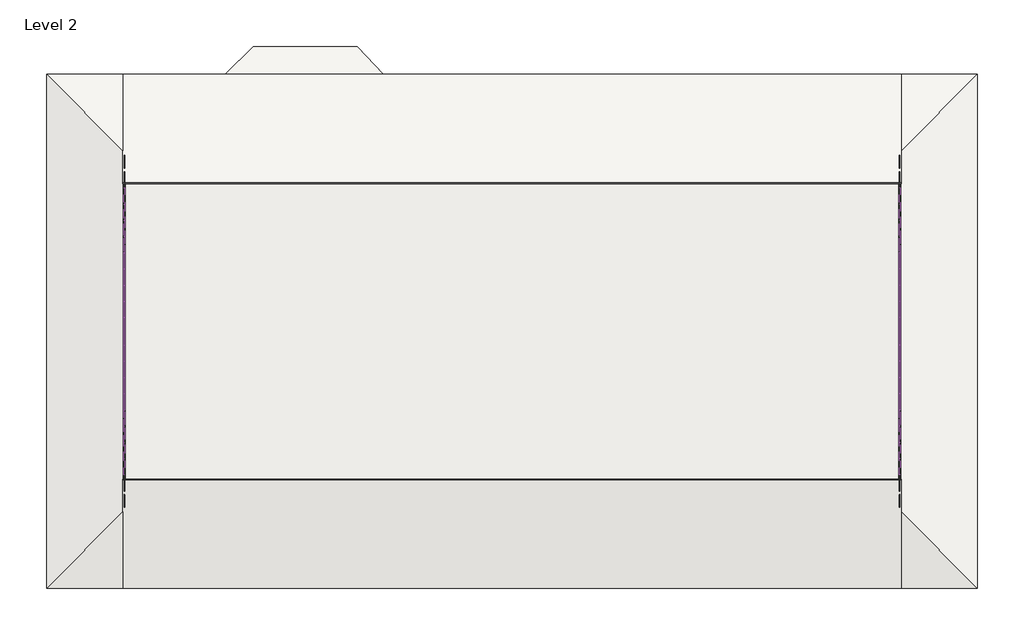
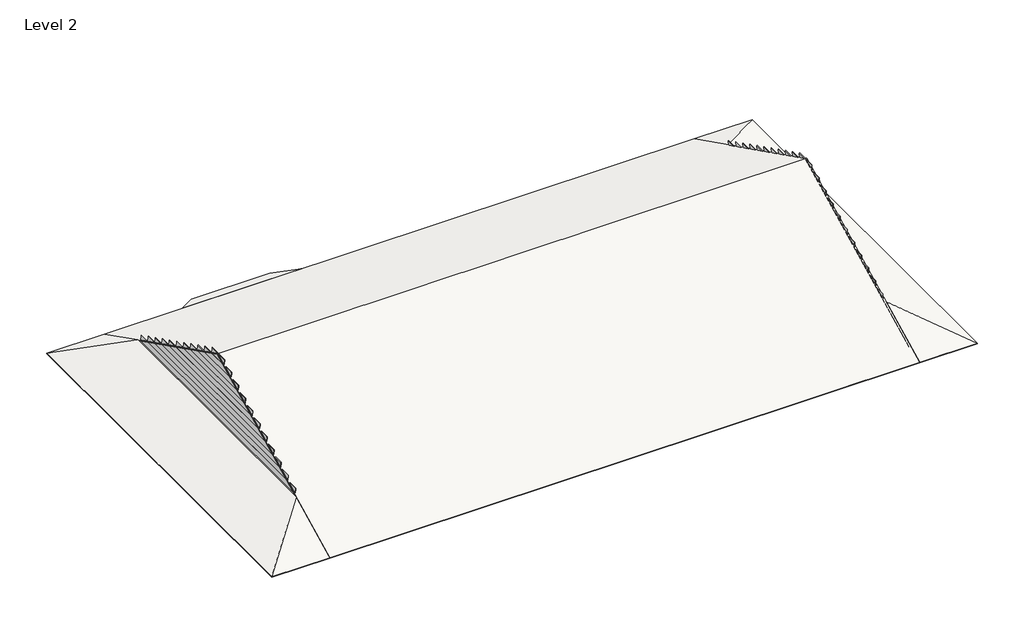
# One storey: 22 proxies, 4 roofs, 2 walls, 1 covering.
"""IFC4 building model written with IfcOpenShell, lengths in millimetres."""

from ifc_helpers import new_model, si_unit, frame, origin, place, context, project, spatial, polyline, outline, extrude, faceted_brep, element, save

model = new_model("IFC4")

# Units and contexts
model_context = context("Model", 3, world=origin())
ifc_project = project(units=[si_unit("LENGTHUNIT", "METRE", prefix="MILLI")], contexts=[model_context])

# Site, building, storey
site = spatial("IfcSite", under=ifc_project)
building = spatial("IfcBuilding", under=site)
storey = spatial("IfcBuildingStorey", under=building, Name="Level 2", Elevation=2768.6)

# Proxies
placement = place(None, origin())
element("IfcBuildingElementProxy", 1, Name="Wall Sweeps", at=placement, inside=storey, context=model_context, shape_type="SweptSolid", body=[
    extrude(outline(polyline([(0.0, -10.0), (0.0, 0.0), (7721.6, 0.0), (7721.6, -10.0), (0.0, -10.0)])), frame((468.8525114, 3886.9284114, 3659.1151454), z_axis=(-0.08859633935570814, 0.0, 0.9960676124906221), x_axis=(0.0, -1.0, 0.0)), (0.0, 0.0, 1.0), 160.0),
])
element("IfcBuildingElementProxy", 2, Name="Wall Sweeps", at=placement, inside=storey, context=model_context, shape_type="SweptSolid", body=[
    extrude(outline(polyline([(0.0, -10.0), (0.0, 0.0), (7010.4, 0.0), (7010.4, -10.0), (0.0, -10.0)])), frame((468.8525114, 3531.3284114, 3836.9151454), z_axis=(-0.08859633935570814, 0.0, 0.9960676124906221), x_axis=(0.0, -1.0, 0.0)), (0.0, 0.0, 1.0), 160.0),
])
element("IfcBuildingElementProxy", 3, Name="Wall Sweeps", at=placement, inside=storey, context=model_context, shape_type="SweptSolid", body=[
    extrude(outline(polyline([(0.0, -10.0), (0.0, 0.0), (6299.2, 0.0), (6299.2, -10.0), (0.0, -10.0)])), frame((468.8525114, 3175.7284114, 4014.7151454), z_axis=(-0.08859633935570814, 0.0, 0.9960676124906221), x_axis=(0.0, -1.0, 0.0)), (0.0, 0.0, 1.0), 160.0),
])
element("IfcBuildingElementProxy", 4, Name="Wall Sweeps", at=placement, inside=storey, context=model_context, shape_type="SweptSolid", body=[
    extrude(outline(polyline([(0.0, -10.0), (0.0, 0.0), (5588.0, 0.0), (5588.0, -10.0), (0.0, -10.0)])), frame((468.8525114, 2820.1284114, 4192.5151454), z_axis=(-0.08859633935570814, 0.0, 0.9960676124906221), x_axis=(0.0, -1.0, 0.0)), (0.0, 0.0, 1.0), 160.0),
])
element("IfcBuildingElementProxy", 5, Name="Wall Sweeps", at=placement, inside=storey, context=model_context, shape_type="SweptSolid", body=[
    extrude(outline(polyline([(0.0, -10.0), (0.0, 0.0), (4876.8, 0.0), (4876.8, -10.0), (0.0, -10.0)])), frame((468.8525114, 2464.5284114, 4370.3151454), z_axis=(-0.08859633935570814, 0.0, 0.9960676124906221), x_axis=(0.0, -1.0, 0.0)), (0.0, 0.0, 1.0), 160.0),
])
element("IfcBuildingElementProxy", 6, Name="Wall Sweeps", at=placement, inside=storey, context=model_context, shape_type="SweptSolid", body=[
    extrude(outline(polyline([(0.0, -10.0), (0.0, 0.0), (4165.6, 0.0), (4165.6, -10.0), (0.0, -10.0)])), frame((468.8525114, 2108.9284114, 4548.1151454), z_axis=(-0.08859633935570814, 0.0, 0.9960676124906221), x_axis=(0.0, -1.0, 0.0)), (0.0, 0.0, 1.0), 160.0),
])
element("IfcBuildingElementProxy", 7, Name="Wall Sweeps", at=placement, inside=storey, context=model_context, shape_type="SweptSolid", body=[
    extrude(outline(polyline([(0.0, -10.0), (0.0, 0.0), (3454.4, 0.0), (3454.4, -10.0), (0.0, -10.0)])), frame((468.8525114, 1753.3284114, 4725.9151454), z_axis=(-0.08859633935570814, 0.0, 0.9960676124906221), x_axis=(0.0, -1.0, 0.0)), (0.0, 0.0, 1.0), 160.0),
])
element("IfcBuildingElementProxy", 8, Name="Wall Sweeps", at=placement, inside=storey, context=model_context, shape_type="SweptSolid", body=[
    extrude(outline(polyline([(0.0, -10.0000001), (0.0, 0.0), (7721.6, 0.0), (7721.6, -10.0000001), (0.0, -10.0000001)])), frame((-16554.1214933, 3886.9284114, 3658.229182), z_axis=(0.08859633935570814, 0.0, 0.9960676124906221), x_axis=(0.0, -1.0, 0.0)), (0.0, 0.0, 1.0), 160.0),
])
element("IfcBuildingElementProxy", 9, Name="Wall Sweeps", at=placement, inside=storey, context=model_context, shape_type="SweptSolid", body=[
    extrude(outline(polyline([(0.0, -10.0000001), (0.0, 0.0), (7010.4, 0.0), (7010.4, -10.0000001), (0.0, -10.0000001)])), frame((-16554.1214933, 3531.3284114, 3836.029182), z_axis=(0.08859633935570814, 0.0, 0.9960676124906221), x_axis=(0.0, -1.0, 0.0)), (0.0, 0.0, 1.0), 160.0),
])
element("IfcBuildingElementProxy", 10, Name="Wall Sweeps", at=placement, inside=storey, context=model_context, shape_type="SweptSolid", body=[
    extrude(outline(polyline([(0.0, -10.0000001), (0.0, 0.0), (6299.2, 0.0), (6299.2, -10.0000001), (0.0, -10.0000001)])), frame((-16554.1214933, 3175.7284114, 4013.829182), z_axis=(0.08859633935570814, 0.0, 0.9960676124906221), x_axis=(0.0, -1.0, 0.0)), (0.0, 0.0, 1.0), 160.0),
])
element("IfcBuildingElementProxy", 11, Name="Wall Sweeps", at=placement, inside=storey, context=model_context, shape_type="SweptSolid", body=[
    extrude(outline(polyline([(0.0, -10.0000001), (0.0, 0.0), (5588.0, 0.0), (5588.0, -10.0000001), (0.0, -10.0000001)])), frame((-16554.1214933, 2820.1284114, 4191.629182), z_axis=(0.08859633935570814, 0.0, 0.9960676124906221), x_axis=(0.0, -1.0, 0.0)), (0.0, 0.0, 1.0), 160.0),
])
element("IfcBuildingElementProxy", 12, Name="Wall Sweeps", at=placement, inside=storey, context=model_context, shape_type="SweptSolid", body=[
    extrude(outline(polyline([(0.0, -10.0000001), (0.0, 0.0), (4876.8, 0.0), (4876.8, -10.0000001), (0.0, -10.0000001)])), frame((-16554.1214933, 2464.5284114, 4369.429182), z_axis=(0.08859633935570814, 0.0, 0.9960676124906221), x_axis=(0.0, -1.0, 0.0)), (0.0, 0.0, 1.0), 160.0),
])
element("IfcBuildingElementProxy", 13, Name="Wall Sweeps", at=placement, inside=storey, context=model_context, shape_type="SweptSolid", body=[
    extrude(outline(polyline([(0.0, -10.0000001), (0.0, 0.0), (4165.6, 0.0), (4165.6, -10.0000001), (0.0, -10.0000001)])), frame((-16554.1214933, 2108.9284114, 4547.229182), z_axis=(0.08859633935570814, 0.0, 0.9960676124906221), x_axis=(0.0, -1.0, 0.0)), (0.0, 0.0, 1.0), 160.0),
])
element("IfcBuildingElementProxy", 14, Name="Wall Sweeps", at=placement, inside=storey, context=model_context, shape_type="SweptSolid", body=[
    extrude(outline(polyline([(0.0, -10.0000001), (0.0, 0.0), (3454.4, 0.0), (3454.4, -10.0000001), (0.0, -10.0000001)])), frame((-16554.1214933, 1753.3284114, 4725.029182), z_axis=(0.08859633935570814, 0.0, 0.9960676124906221), x_axis=(0.0, -1.0, 0.0)), (0.0, 0.0, 1.0), 160.0),
])
element("IfcBuildingElementProxy", 15, Name="Wall Sweeps", at=placement, inside=storey, context=model_context, shape_type="SweptSolid", body=[
    extrude(outline(polyline([(0.0, -10.0), (0.0, 0.0), (2743.2, 0.0), (2743.2, -10.0), (0.0, -10.0)])), frame((468.8525114, 1397.7284114, 4903.7151454), z_axis=(-0.08859633935570814, 0.0, 0.9960676124906221), x_axis=(0.0, -1.0, 0.0)), (0.0, 0.0, 1.0), 160.0),
])
element("IfcBuildingElementProxy", 16, Name="Wall Sweeps", at=placement, inside=storey, context=model_context, shape_type="SweptSolid", body=[
    extrude(outline(polyline([(0.0, -10.0), (0.0, 0.0), (2032.0, 0.0), (2032.0, -10.0), (0.0, -10.0)])), frame((468.8525114, 1042.1284114, 5081.5151454), z_axis=(-0.08859633935570814, 0.0, 0.9960676124906221), x_axis=(0.0, -1.0, 0.0)), (0.0, 0.0, 1.0), 160.0),
])
element("IfcBuildingElementProxy", 17, Name="Wall Sweeps", at=placement, inside=storey, context=model_context, shape_type="SweptSolid", body=[
    extrude(outline(polyline([(0.0, -10.0), (0.0, 0.0), (1320.8, 0.0), (1320.8, -10.0), (0.0, -10.0)])), frame((468.8525114, 686.5284114, 5259.3151454), z_axis=(-0.08859633935570814, 0.0, 0.9960676124906221), x_axis=(0.0, -1.0, 0.0)), (0.0, 0.0, 1.0), 160.0),
])
element("IfcBuildingElementProxy", 18, Name="Wall Sweeps", at=placement, inside=storey, context=model_context, shape_type="SweptSolid", body=[
    extrude(outline(polyline([(0.0, -10.0), (0.0, 0.0), (609.6, 0.0), (609.6, -10.0), (0.0, -10.0)])), frame((468.8525114, 330.9284114, 5437.1151454), z_axis=(-0.08859633935570814, 0.0, 0.9960676124906221), x_axis=(0.0, -1.0, 0.0)), (0.0, 0.0, 1.0), 160.0),
])
element("IfcBuildingElementProxy", 19, Name="Wall Sweeps", at=placement, inside=storey, context=model_context, shape_type="SweptSolid", body=[
    extrude(outline(polyline([(0.0, -10.0000001), (0.0, 0.0), (2743.2, 0.0), (2743.2, -10.0000001), (0.0, -10.0000001)])), frame((-16554.1214933, 1397.7284114, 4902.829182), z_axis=(0.08859633935570814, 0.0, 0.9960676124906221), x_axis=(0.0, -1.0, 0.0)), (0.0, 0.0, 1.0), 160.0),
])
element("IfcBuildingElementProxy", 20, Name="Wall Sweeps", at=placement, inside=storey, context=model_context, shape_type="SweptSolid", body=[
    extrude(outline(polyline([(0.0, -10.0000001), (0.0, 0.0), (2032.0, 0.0), (2032.0, -10.0000001), (0.0, -10.0000001)])), frame((-16554.1214933, 1042.1284114, 5080.629182), z_axis=(0.08859633935570814, 0.0, 0.9960676124906221), x_axis=(0.0, -1.0, 0.0)), (0.0, 0.0, 1.0), 160.0),
])
element("IfcBuildingElementProxy", 21, Name="Wall Sweeps", at=placement, inside=storey, context=model_context, shape_type="SweptSolid", body=[
    extrude(outline(polyline([(0.0, -10.0000001), (0.0, 0.0), (1320.8, 0.0), (1320.8, -10.0000001), (0.0, -10.0000001)])), frame((-16554.1214933, 686.5284114, 5258.429182), z_axis=(0.08859633935570814, 0.0, 0.9960676124906221), x_axis=(0.0, -1.0, 0.0)), (0.0, 0.0, 1.0), 160.0),
])
element("IfcBuildingElementProxy", 22, Name="Wall Sweeps", at=placement, inside=storey, context=model_context, shape_type="SweptSolid", body=[
    extrude(outline(polyline([(0.0, -10.0000001), (0.0, 0.0), (609.6, 0.0), (609.6, -10.0000001), (0.0, -10.0000001)])), frame((-16554.1214933, 330.9284114, 5436.229182), z_axis=(0.08859633935570814, 0.0, 0.9960676124906221), x_axis=(0.0, -1.0, 0.0)), (0.0, 0.0, 1.0), 160.0),
])

# Covering
element("IfcCovering", 23, ObjectType="BLDG 6241 celling", at=placement, inside=storey, context=model_context, shape_type="SweptSolid", body=[
    extrude(outline(polyline([(-17801.214829, -5060.2215886), (-17801.214829, 5207.7284114), (-13999.9307311, 5207.7284114), (-13542.7307311, 5664.9284114), (-11675.456878, 5664.9284114), (-11218.256878, 5207.7284114), (1705.985171, 5207.7284114), (1705.985171, -5053.8715886), (1705.985171, -5155.4715886), (-5609.214829, -5155.4715886), (-5609.214829, -5053.8715886), (-5609.214829, -3631.4715886), (-7438.014829, -3631.4715886), (-7438.014829, -5060.2215886), (-17801.214829, -5060.2215886)])), frame((0.0, 0.0, 2768.6), z_axis=(0.0, 0.0, 1.0), x_axis=(1.0, 0.0, 0.0)), (0.0, 0.0, 1.0), 12.7),
])

# Roofs
element("IfcRoof", 24, ObjectType="Generic - 12\"", at=placement, inside=storey, context=model_context, shape_type="Brep", body=[
    faceted_brep([(-5609.214829, -5612.6715886, 2768.6), (-5609.214829, -5612.6715886, 2784.5739106), (-16582.014829, -5612.6715886, 2784.5739106), (-16582.014829, -5612.6715886, 2768.6), (486.785171, -5612.6715886, 2768.6), (486.785171, -5612.6715886, 2784.5739106), (-16582.014829, 5664.9284114, 2768.6), (486.785171, 5664.9284114, 2768.6), (486.785171, 26.1284114, 5588.0), (-16582.014829, 26.1284114, 5588.0), (486.785171, 5664.9284114, 2784.5739106), (-16582.014829, 5664.9284114, 2784.5739106), (-16582.014829, 26.1284114, 5603.9739106), (486.785171, 26.1284114, 5603.9739106)], [[[0, 1, 2, 3]], [[4, 5, 1, 0]], [[6, 7, 8, 9]], [[10, 11, 12, 13]], [[6, 11, 10, 7]], [[8, 4, 0, 3, 9]], [[5, 13, 12, 2, 1]], [[10, 13, 5, 4, 8, 7]], [[2, 12, 11, 6, 9, 3]]]),
])
element("IfcRoof", 25, ObjectType="Generic - 12\"", at=placement, inside=storey, context=model_context, shape_type="Brep", body=[
    faceted_brep([(-14332.9932698, 5664.9284114, 2768.6), (-13723.3932698, 6274.5284114, 2463.8), (-11443.0667952, 6274.5284114, 2463.8), (-10875.5508932, 5664.9284114, 2768.6), (-13723.3932698, 6274.5284114, 2479.7739106), (-14332.9932698, 5664.9284114, 2784.5739106), (-10875.5508932, 5664.9284114, 2784.5739106), (-11443.0667952, 6274.5284114, 2479.7739106)], [[[0, 1, 2, 3]], [[4, 5, 6, 7]], [[1, 4, 7, 2]], [[5, 4, 1, 0]], [[7, 6, 3, 2]], [[6, 5, 0, 3]]]),
])
element("IfcRoof", 26, ObjectType="Generic - 12\"", at=placement, inside=storey, context=model_context, shape_type="Brep", body=[
    faceted_brep([(-18258.414829, 5664.9284114, 2768.6), (-16582.014829, 3988.5284114, 3606.8), (-16582.014829, -3936.2715886, 3606.8), (-18258.414829, -5612.6715886, 2768.6), (-18258.414829, 5664.9284114, 2784.5739106), (-18258.414829, -5612.6715886, 2784.5739106), (-16582.014829, -3936.2715886, 3622.7739106), (-16582.014829, 3988.5284114, 3622.7739106), (-16582.014829, 5664.9284114, 2768.6), (-16582.014829, -5612.6715886, 2768.6), (-16582.014829, 5664.9284114, 2784.5739106), (-16582.014829, -5612.6715886, 2784.5739106)], [[[0, 1, 2, 3]], [[4, 5, 6, 7]], [[3, 5, 4, 0]], [[0, 8, 1]], [[2, 9, 3]], [[10, 4, 7]], [[11, 6, 5]], [[0, 4, 10, 8]], [[9, 11, 5, 3]], [[10, 7, 6, 11, 9, 2, 1, 8]]]),
])
element("IfcRoof", 27, ObjectType="Generic - 12\"", at=placement, inside=storey, context=model_context, shape_type="Brep", body=[
    faceted_brep([(486.785171, 3988.5284114, 3606.8), (486.785171, 5664.9284114, 2768.6), (2163.185171, 5664.9284114, 2768.6), (2163.185171, -5612.6715886, 2768.6), (486.785171, -3936.2715886, 3606.8), (486.785171, -5612.6715886, 2768.6), (486.785171, 5664.9284114, 2784.5739106), (486.785171, 3988.5284114, 3622.7739106), (2163.185171, 5664.9284114, 2784.5739106), (2163.185171, -5612.6715886, 2784.5739106), (486.785171, -3936.2715886, 3622.7739106), (486.785171, -5612.6715886, 2784.5739106)], [[[0, 1, 2]], [[3, 4, 0, 2]], [[3, 5, 4]], [[6, 7, 8]], [[9, 8, 7, 10]], [[11, 9, 10]], [[1, 6, 8, 2]], [[3, 9, 11, 5]], [[2, 8, 9, 3]], [[11, 10, 7, 6, 1, 0, 4, 5]]]),
])

# Walls
element("IfcWall", 28, ObjectType="BLDG 6241 ROOF 2", at=placement, inside=storey, context=model_context, shape_type="SweptSolid", body=[
    extrude(outline(polyline([(5106.1284114, 2768.6), (-5155.4715886, 2768.6), (-5155.4715886, 2997.2), (26.1284114, 5588.0), (5106.1284114, 3048.0), (5106.1284114, 2768.6)])), frame((433.603921, 0.0, 0.0), z_axis=(1.0, 0.0, 0.0), x_axis=(0.0, 1.0, 0.0)), (0.0, 0.0, 1.0), 11.1125),
])
element("IfcWall", 29, ObjectType="BLDG 6241 ROOF 3", at=placement, inside=storey, context=model_context, shape_type="SweptSolid", body=[
    extrude(outline(polyline([(5106.1284114, 2768.6), (-5053.8715886, 2768.6), (-5053.8715886, 3048.0), (26.1284114, 5588.0), (5106.1284114, 3048.0), (5106.1284114, 2768.6)])), frame((-16539.946079, 0.0, 0.0), z_axis=(1.0, 0.0, 0.0), x_axis=(0.0, 1.0, 0.0)), (0.0, 0.0, 1.0), 11.1125),
])

save(model, "model.ifc")

# Revit data of these elements
# Type "BLDG 6241 celling"
#   Assembly Code = "C3030210"
#   built-in parameter 1002203 = 1 (stored number, unit not read)
#   built-in parameter 1002202 = 1 (stored number, unit not read)
#   Layers, outside or top first: 0' - 0 1/2" "Gypsum Wall Board" (function 4)
# Type "Generic - 12\""
#   Assembly Code = "B1020"
#   Layers, outside or top first: 0' - 0 1/8" "BLDG 6241 roof" (function 5); 0' - 0" "Asphalt Shingle" (function 100); 0' - 0 7/16" "BLDG 6241 23/32\" OSB board" (function 4)
# Type "BLDG 6241 ROOF 2"
#   Assembly Code = "B2010"
#   Layers, outside or top first: 0' - 0 7/16" "BLDG 6241 23/32\" OSB board" (function 4)
# Type "BLDG 6241 ROOF 3"
#   Assembly Code = "B2010"
#   Layers, outside or top first: 0' - 0 7/16" "BLDG 6241 23/32\" OSB board" (function 4)
# Elements 1, 2, 3, 4, 5, 6, 7, 8, 9, 10, 11, 12, 13, 14, 15, 16, 17, 18, 19, 20, 21, 22 (IfcBuildingElementProxy)
#   Phase Created = New Construction
#   Materials on its faces: "Aluminum"
# Element 23 (IfcCovering, "BLDG 6241 celling")
#   Height Offset From Level = 0' - 0"
#   Phase Created = New Construction
#   Materials on its faces: "Gypsum Wall Board"
# Element 24 (IfcRoof, "Generic - 12\"")
#   built-in parameter 1001705 = 18.3857 (stored number, unit not read)
#   built-in parameter 1001710 = 33615
#   Phase Created = New Construction
#   Materials on its faces: "BLDG 6241 23/32\" OSB board", "BLDG 6241 roof"
# Element 25 (IfcRoof, "Generic - 12\"")
#   built-in parameter 1001705 = 9.13574 (stored number, unit not read)
#   built-in parameter 1001701 = -1 (stored number, unit not read)
#   built-in parameter 1001710 = 33615
#   Phase Created = New Construction
#   Materials on its faces: "BLDG 6241 23/32\" OSB board", "BLDG 6241 roof"
# Elements 26, 27 (IfcRoof, "Generic - 12\"")
#   built-in parameter 1001705 = 11.8857 (stored number, unit not read)
#   built-in parameter 1001710 = 33615
#   Phase Created = New Construction
#   Materials on its faces: "BLDG 6241 23/32\" OSB board", "BLDG 6241 roof"
# Element 28 (IfcWall, "BLDG 6241 ROOF 2")
#   Top Offset = 0' - 0"
#   Base Offset = 0' - 0"
#   Unconnected Height = 9' - 1"
#   wall height = 9' - 1"
#   Phase Created = New Construction
#   Base Constraint = Level 2
#   Materials on its faces: "BLDG 6241 23/32\" OSB board"
# Element 29 (IfcWall, "BLDG 6241 ROOF 3")
#   Top Offset = 0' - 0"
#   Base Offset = 0' - 0"
#   Unconnected Height = 9' - 1"
#   wall height = 9' - 1"
#   Phase Created = New Construction
#   Base Constraint = Level 2
#   Materials on its faces: "BLDG 6241 23/32\" OSB board"
# Materials
#   "Gypsum Wall Board": class "Generic", colour RGB 127 127 127, transparency 0, Description = "Gypsum Wall Board", Cost = 0
#   "BLDG 6241 roof": class "Generic", colour RGB 85 51 38, transparency 0, Description = "BLDG 6241 roof", Cost = 0
#   "Asphalt Shingle": class "Generic", colour RGB 155 155 155, transparency 0, Description = "Asphalt roofing shingle", Cost = 0
#   "BLDG 6241 23/32\" OSB board": class "Generic", colour RGB 193 140 64, transparency 0, Description = "BLDG 6241 23/32\" OSB board", Cost = 0
#   "Aluminum": class "Metal", colour RGB 244 244 244, transparency 0, Description = "Aluminum 6061", Cost = 0
